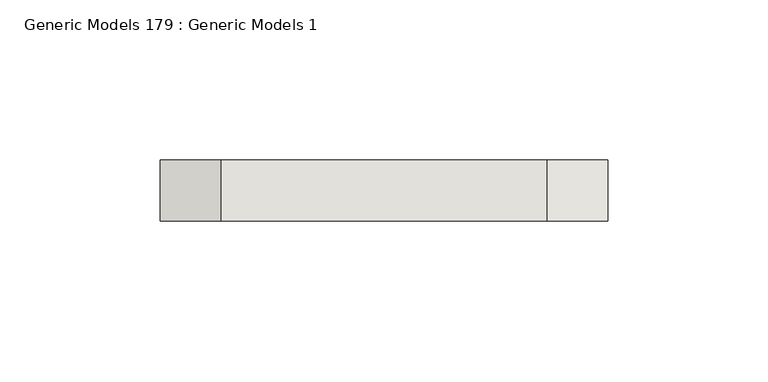
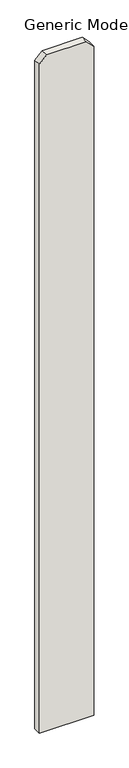
"""IFC4 building model written with IfcOpenShell, lengths in millimetres: wall geometry, Generic Models 179 : Generic Models 1."""

from ifc_helpers import new_model, si_unit, frame, origin, place, context, project, spatial, polyline, outline, extrude, source, transform, mapped, element, save


def generic_models_179_generic_models_1_e8752753(model_context):
    return source(origin(), model_context, "Body", "SweptSolid", [
        extrude(outline(polyline([(76.2, 325956.6125), (1885.95, 325956.6125), (1905.0, 325937.5625), (1905.0, 325835.9625), (1885.95, 325816.9125), (76.2, 325816.9125), (76.2, 325956.6125)])), frame((0.0, 547.6875, 0.0), z_axis=(0.0, 1.0, 0.0), x_axis=(0.0, 0.0, 1.0)), (0.0, 0.0, 1.0), 19.05),
    ])


if __name__ == "__main__":
    model = new_model("IFC4")
    model_context = context("Model", 3, world=origin())
    ifc_project = project(units=[si_unit("LENGTHUNIT", "METRE", prefix="MILLI")], contexts=[model_context])
    site = spatial("IfcSite", under=ifc_project)
    building = spatial("IfcBuilding", under=site)
    placement = place(None, origin())
    generic_models_179_generic_models_1_shape = generic_models_179_generic_models_1_e8752753(model_context)
    element("IfcWall", 1, ObjectType="Generic Models 179 : Generic Models 1", at=placement, inside=building, context=model_context, shape_type="MappedRepresentation", body=[
        mapped(generic_models_179_generic_models_1_shape, transform((0.0, 0.0, 0.0), x_axis=(1.0, 0.0, 0.0), y_axis=(0.0, 1.0, 0.0), z_axis=(0.0, 0.0, 1.0))),
    ])
    save(model, "model.ifc")

# Revit data of these elements
# Element 1 (IfcWall, "Generic Models 179 : Generic Models 1")
#   Materials on its faces: "VERTICAL 1X6 CEDAR PLANKS W/ CLEAR WOOD SEALER"
# Materials
#   "VERTICAL 1X6 CEDAR PLANKS W/ CLEAR WOOD SEALER": class "Wood", colour RGB 234 198 147, transparency 0, Description = "Pinus Echinata", Cost = 0
